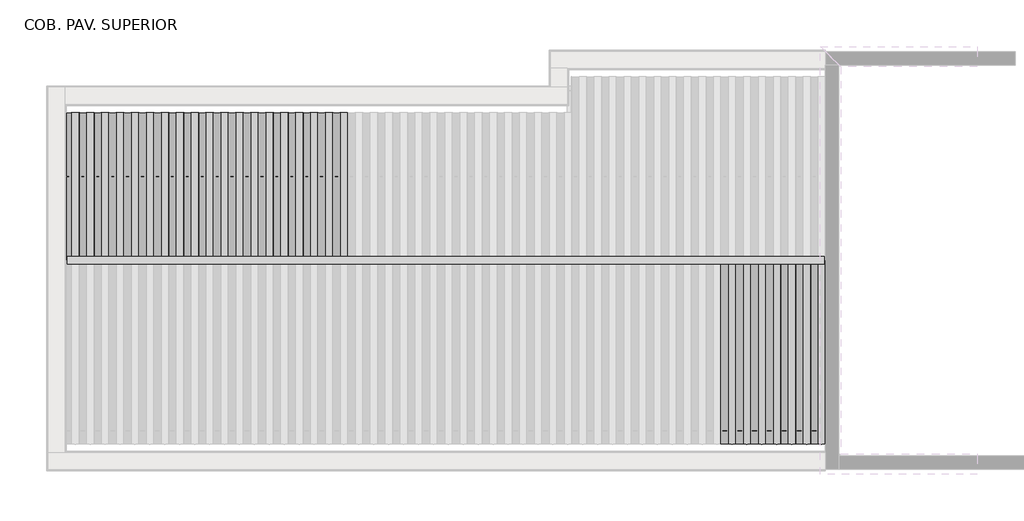
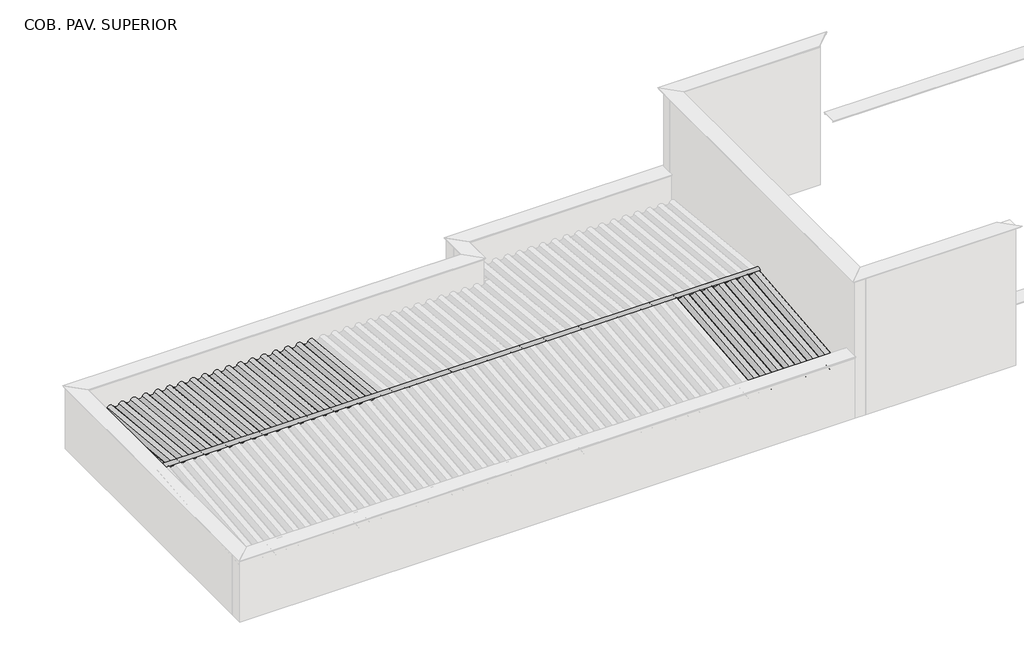
# One storey, part 3 of 7: 37 beams, 7 columns.
"""IFC4 building model written with IfcOpenShell, lengths in millimetres."""

import ifcopenshell
import ifcopenshell.guid

model = None  # the IFC model being written
_history = None  # IfcOwnerHistory: only IFC2X3 demands one
_inside = {}  # id of a spatial element -> (the spatial element, [elements in it])
_under = {}  # id of a project, library or spatial element -> (it, [spatial elements below it])
_declared = {}  # id of a project -> (the project, [libraries it declares])
_typed = {}  # id of a type object -> (the type object, [elements of that type])
_made_of = {}  # id of a material, layer set ... -> (it, [elements and type objects made of it])


def new_model(schema):
    """Start an empty IFC model of exactly this schema.

    Asked for "IFC4X3", IfcOpenShell would pick the latest addendum, in which some entities
    have other attributes; the version numbers below select the first issue.
    IFC2X3 requires an IfcOwnerHistory on every rooted entity: one is made here for all.
    """
    global model, _history
    if schema == "IFC4X3":
        model = ifcopenshell.file(schema_version=(4, 3, 0, 0))
    else:
        model = ifcopenshell.file(schema=schema)
    _inside.clear()
    _under.clear()
    _declared.clear()
    _typed.clear()
    _made_of.clear()
    _history = None
    if model.schema == "IFC2X3":
        org = make("IfcOrganization", Name="unknown")
        user = make(
            "IfcPersonAndOrganization",
            ThePerson=make("IfcPerson", FamilyName="unknown"),
            TheOrganization=org,
        )
        app = make(
            "IfcApplication",
            ApplicationDeveloper=org,
            Version="unknown",
            ApplicationFullName="unknown",
            ApplicationIdentifier="unknown",
        )
        _history = make(
            "IfcOwnerHistory",
            OwningUser=user,
            OwningApplication=app,
            ChangeAction="ADDED",
            CreationDate=0,
        )
    return model


def make(cls, **values):
    """One entity of the class cls with the attributes given. An attribute that is None is left unset."""
    return model.create_entity(
        cls, **{name: value for name, value in values.items() if value is not None}
    )


def rooted(cls, **values):
    """An entity with a GlobalId (a new one), such as an element, a storey or a relation."""
    return make(cls, GlobalId=ifcopenshell.guid.new(), OwnerHistory=_history, **values)


def si_unit(unit_type, name, prefix=None):
    """IfcSIUnit, for example si_unit("LENGTHUNIT", "METRE", prefix="MILLI")."""
    return make("IfcSIUnit", UnitType=unit_type, Prefix=prefix, Name=name)


def assignment(units):
    """IfcUnitAssignment: the units of a project."""
    return None if units is None else make("IfcUnitAssignment", Units=units)


def point(xyz):
    """IfcCartesianPoint."""
    return None if xyz is None else make("IfcCartesianPoint", Coordinates=xyz)


def direction(xyz):
    """IfcDirection."""
    return None if xyz is None else make("IfcDirection", DirectionRatios=xyz)


def frame(location, z_axis=None, x_axis=None):
    """IfcAxis2Placement3D, a coordinate frame: its origin and axes. An axis left out is left unset."""
    return make(
        "IfcAxis2Placement3D",
        Location=point(location),
        Axis=direction(z_axis),
        RefDirection=direction(x_axis),
    )


def frame_2d(location, x_axis=None):
    """IfcAxis2Placement2D, a coordinate frame in the plane: its origin and x axis."""
    return make(
        "IfcAxis2Placement2D", Location=point(location), RefDirection=direction(x_axis)
    )


def origin():
    """The frame at (0, 0, 0) with its axes left unset."""
    return frame((0.0, 0.0, 0.0))


def place(relative_to, where):
    """IfcLocalPlacement: puts the frame where relative to a parent placement (None: the world)."""
    return make(
        "IfcLocalPlacement", PlacementRelTo=relative_to, RelativePlacement=where
    )


def context(
    kind, dimensions, precision=None, world=None, true_north=None, identifier=None
):
    """IfcGeometricRepresentationContext, for example the 3D "Model" context."""
    return make(
        "IfcGeometricRepresentationContext",
        ContextIdentifier=identifier,
        ContextType=kind,
        CoordinateSpaceDimension=dimensions,
        Precision=precision,
        WorldCoordinateSystem=world,
        TrueNorth=true_north,
    )


def project(units=None, contexts=None):
    """IfcProject with its units and contexts."""
    return rooted(
        "IfcProject",
        Name="project",
        RepresentationContexts=contexts,
        UnitsInContext=assignment(units),
    )


def spatial(cls, under=None, at=None, **own):
    """A site, building, storey or space (cls), placed at a placement, below another one or the project."""
    s = rooted(cls, ObjectPlacement=at, **own)
    if under is not None:
        _under.setdefault(under.id(), (under, []))[1].append(s)
    return s


def polyline(points):
    """IfcPolyline through the points."""
    return make("IfcPolyline", Points=[point(p) for p in points])


def circle_curve(where, radius):
    """IfcCircle in the frame where."""
    return make("IfcCircle", Position=where, Radius=radius)


def trimmed(basis, trim1, trim2, sense, master):
    """IfcTrimmedCurve: the piece of a basis curve between two trims."""
    return make(
        "IfcTrimmedCurve",
        BasisCurve=basis,
        Trim1=trim1,
        Trim2=trim2,
        SenseAgreement=sense,
        MasterRepresentation=master,
    )


def segment(curve, same_sense, transition):
    """IfcCompositeCurveSegment."""
    return make(
        "IfcCompositeCurveSegment",
        Transition=transition,
        SameSense=same_sense,
        ParentCurve=curve,
    )


def composite_curve(segments, self_intersect=None):
    """IfcCompositeCurve: segments joined end to end."""
    return make("IfcCompositeCurve", Segments=segments, SelfIntersect=self_intersect)


def outline(outer, holes=None, kind="AREA"):
    """IfcArbitraryClosedProfileDef: a profile drawn as a closed curve; with holes, ...WithVoids."""
    if holes is None:
        return make("IfcArbitraryClosedProfileDef", ProfileType=kind, OuterCurve=outer)
    return make(
        "IfcArbitraryProfileDefWithVoids",
        ProfileType=kind,
        OuterCurve=outer,
        InnerCurves=holes,
    )


def extrude(swept, where, along, depth):
    """IfcExtrudedAreaSolid: the profile swept, set in the frame where, extruded along a direction by depth."""
    return make(
        "IfcExtrudedAreaSolid",
        SweptArea=swept,
        Position=where,
        ExtrudedDirection=direction(along),
        Depth=depth,
    )


def shape(context_of_items, identifier, shape_type, items):
    """IfcShapeRepresentation: the items that make up one representation, for example the "Body"."""
    return make(
        "IfcShapeRepresentation",
        ContextOfItems=context_of_items,
        RepresentationIdentifier=identifier,
        RepresentationType=shape_type,
        Items=items,
    )


def source(mapping_origin, context_of_items, identifier, shape_type, items):
    """IfcRepresentationMap: a shape defined once, which mapped items show again and again."""
    return make(
        "IfcRepresentationMap",
        MappingOrigin=mapping_origin,
        MappedRepresentation=shape(context_of_items, identifier, shape_type, items),
    )


def transform(
    local_origin,
    x_axis=None,
    y_axis=None,
    z_axis=None,
    scale=None,
    scale2=None,
    scale3=None,
    uniform=True,
):
    """IfcCartesianTransformationOperator3D, or its non-uniform kind. x_axis, y_axis, z_axis: its Axis1, 2, 3."""
    if uniform:
        return make(
            "IfcCartesianTransformationOperator3D",
            Axis1=direction(x_axis),
            Axis2=direction(y_axis),
            LocalOrigin=point(local_origin),
            Scale=scale,
            Axis3=direction(z_axis),
        )
    return make(
        "IfcCartesianTransformationOperator3DnonUniform",
        Axis1=direction(x_axis),
        Axis2=direction(y_axis),
        LocalOrigin=point(local_origin),
        Scale=scale,
        Axis3=direction(z_axis),
        Scale2=scale2,
        Scale3=scale3,
    )


def mapped(mapping_source, mapping_target):
    """IfcMappedItem: shows the shape of a source again, moved by a transform."""
    return make(
        "IfcMappedItem", MappingSource=mapping_source, MappingTarget=mapping_target
    )


def made_of(thing, what):
    """Note that an element or type object is made of a material, layer set ...; save() writes the relation."""
    if what is not None:
        _made_of.setdefault(what.id(), (what, []))[1].append(thing)
    return thing


def element(
    cls,
    number,
    at=None,
    inside=None,
    cuts=None,
    type_object=None,
    material=None,
    context=None,
    identifier="Body",
    shape_type=None,
    held_by="IfcProductDefinitionShape",
    body=None,
    shapes=None,
    **own,
):
    """One element of the class cls, such as IfcWall. Its Tag is "e" and its number.

    at: its placement. inside: the storey or other place that contains it. cuts: it is an
    opening in that element (IfcRelVoidsElement). A single representation is given by context,
    identifier, shape_type and body (its items); several are given by shapes. held_by: the class
    of the entity that holds the representations. save() writes the other relations.
    """
    e = rooted(cls, Tag="e%d" % number, ObjectPlacement=at, **own)
    if body is not None:
        shapes = [shape(context, identifier, shape_type, body)]
    if shapes is not None:
        e.Representation = make(held_by, Representations=shapes)
    if inside is not None:
        _inside.setdefault(inside.id(), (inside, []))[1].append(e)
    if cuts is not None:
        rooted(
            "IfcRelVoidsElement", RelatingBuildingElement=cuts, RelatedOpeningElement=e
        )
    if type_object is not None:
        _typed.setdefault(type_object.id(), (type_object, []))[1].append(e)
    return made_of(e, material)


def aggregate(whole, parts):
    """IfcRelAggregates: a whole, such as a stair, and the parts it consists of."""
    return rooted("IfcRelAggregates", RelatingObject=whole, RelatedObjects=parts)


def save(model, path):
    """Write the relations noted so far, then the file.

    IfcRelAggregates (storeys below a building ...), IfcRelContainedInSpatialStructure (elements
    in a storey), IfcRelDefinesByType, IfcRelAssociatesMaterial and IfcRelDeclares: one each for
    every whole, place, type object, material and project.
    """
    for whole, parts in _under.values():
        aggregate(whole, parts)
    for where, things in _inside.values():
        rooted(
            "IfcRelContainedInSpatialStructure",
            RelatedElements=things,
            RelatingStructure=where,
        )
    for kind, things in _typed.values():
        rooted("IfcRelDefinesByType", RelatedObjects=things, RelatingType=kind)
    for what, things in _made_of.values():
        rooted("IfcRelAssociatesMaterial", RelatedObjects=things, RelatingMaterial=what)
    for by, libraries in _declared.values():
        rooted("IfcRelDeclares", RelatingContext=by, RelatedDefinitions=libraries)
    model.write(path)


def cumeeira_telha_ondulada_fibrocimento_4a9e66c1(model_context):
    return source(origin(), model_context, "Body", "SweptSolid", [
        extrude(outline(composite_curve([segment(polyline([(58.3970135, 42.4437972), (53.9055884, 40.2467307)]), True, "CONTINUOUS"), segment(trimmed(circle_curve(frame_2d((-1.6029865, 13.0936483)), 61.7939461), [point((53.9055884, 40.2467307))], [point((-57.1115615, 40.2467307))], True, "CARTESIAN"), True, "CONTINUOUS"), segment(polyline([(-57.1115615, 40.2467307), (-61.6029865, 42.4437972)]), True, "CONTINUOUS"), segment(trimmed(circle_curve(frame_2d((-1.6029865, 13.0936483)), 66.7939461), [point((-61.6029865, 42.4437972))], [point((58.3970135, 42.4437972))], False, "CARTESIAN"), True, "CONTINUOUS")], self_intersect=False)), frame((-6200.0, 0.0, 0.0), z_axis=(1.0, 0.0, 0.0), x_axis=(0.0, 1.0, 0.0)), (0.0, 0.0, 1.0), 12400.0),
    ])


def viga_cumeeira_6x16cm_b61bb166(model_context):
    return source(origin(), model_context, "Body", "SweptSolid", [
        extrude(outline(polyline([(6210.0, 30.0), (6210.0, -30.0), (-6210.0, -30.0), (-6210.0, 30.0), (6210.0, 30.0)])), frame((0.0, 0.0, -80.0), z_axis=(0.0, 0.0, 1.0), x_axis=(1.0, 0.0, 0.0)), (0.0, 0.0, 1.0), 160.0),
    ])


def column_d505325c(model_context):
    return source(origin(), model_context, "Body", "SweptSolid", [
        extrude(outline(polyline([(30.0, 80.0), (30.0, -80.0), (-30.0, -80.0), (-30.0, 80.0), (30.0, 80.0)])), frame((0.0, 0.0, 6710.0), z_axis=(0.0, 0.0, 1.0), x_axis=(1.0, 0.0, 0.0)), (0.0, 0.0, 1.0), 750.0),
    ])


def column_df674f92(model_context):
    return source(origin(), model_context, "Body", "SweptSolid", [
        extrude(outline(polyline([(30.0, 80.0), (30.0, -80.0), (-30.0, -80.0), (-30.0, 80.0), (30.0, 80.0)])), frame((0.0, 0.0, 6710.0), z_axis=(0.0, 0.0, 1.0), x_axis=(1.0, 0.0, 0.0)), (0.0, 0.0, 1.0), 575.0),
    ])


def column_4db371bd(model_context):
    return source(origin(), model_context, "Body", "SweptSolid", [
        extrude(outline(polyline([(30.0, 80.0), (30.0, -80.0), (-30.0, -80.0), (-30.0, 80.0), (30.0, 80.0)])), frame((0.0, 0.0, 6710.0), z_axis=(0.0, 0.0, 1.0), x_axis=(1.0, 0.0, 0.0)), (0.0, 0.0, 1.0), 660.0),
    ])


model = new_model("IFC4")

# Units and contexts
model_context = context("Model", 3, world=origin())
ifc_project = project(units=[si_unit("LENGTHUNIT", "METRE", prefix="MILLI")], contexts=[model_context])

# Site, building, storey
site = spatial("IfcSite", under=ifc_project)
building = spatial("IfcBuilding", under=site)
storey = spatial("IfcBuildingStorey", under=building, Name="COB. PAV. SUPERIOR", Elevation=6650.0)

# Beams
placement = place(None, origin())
element("IfcBeam", 1, ObjectType="Madeira de lei : Berço 6x12cm", at=placement, inside=storey, context=model_context, shape_type="SweptSolid", body=[
    extrude(outline(polyline([(-10679.281307, -7711.5607799), (-10679.281307, -7831.5607799), (-12679.281307, -7831.5607799), (-12679.281307, -7711.5607799), (-10679.281307, -7711.5607799)])), frame((0.0, 0.0, 6650.0), z_axis=(0.0, 0.0, 1.0), x_axis=(1.0, 0.0, 0.0)), (0.0, 0.0, 1.0), 60.0),
])
element("IfcBeam", 2, ObjectType="Madeira de lei : Berço 6x12cm", at=placement, inside=storey, context=model_context, shape_type="SweptSolid", body=[
    extrude(outline(polyline([(-8679.281307, -7711.5607799), (-8679.281307, -7831.5607799), (-10679.281307, -7831.5607799), (-10679.281307, -7711.5607799), (-8679.281307, -7711.5607799)])), frame((0.0, 0.0, 6650.0), z_axis=(0.0, 0.0, 1.0), x_axis=(1.0, 0.0, 0.0)), (0.0, 0.0, 1.0), 60.0),
])
element("IfcBeam", 3, ObjectType="Madeira de lei : Berço 6x12cm", at=placement, inside=storey, context=model_context, shape_type="SweptSolid", body=[
    extrude(outline(polyline([(-6679.281307, -7711.5607799), (-6679.281307, -7831.5607799), (-8679.281307, -7831.5607799), (-8679.281307, -7711.5607799), (-6679.281307, -7711.5607799)])), frame((0.0, 0.0, 6650.0), z_axis=(0.0, 0.0, 1.0), x_axis=(1.0, 0.0, 0.0)), (0.0, 0.0, 1.0), 60.0),
])
element("IfcBeam", 4, ObjectType="Madeira de lei : Berço 6x12cm", at=placement, inside=storey, context=model_context, shape_type="SweptSolid", body=[
    extrude(outline(polyline([(-10679.281307, -6319.8711004), (-10679.281307, -6439.8711004), (-12679.281307, -6439.8711004), (-12679.281307, -6319.8711004), (-10679.281307, -6319.8711004)])), frame((0.0, 0.0, 6650.0), z_axis=(0.0, 0.0, 1.0), x_axis=(1.0, 0.0, 0.0)), (0.0, 0.0, 1.0), 60.0),
])
element("IfcBeam", 5, ObjectType="Madeira de lei : Berço 6x12cm", at=placement, inside=storey, context=model_context, shape_type="SweptSolid", body=[
    extrude(outline(polyline([(-10679.281307, -5488.3211004), (-10679.281307, -5608.3211004), (-12679.281307, -5608.3211004), (-12679.281307, -5488.3211004), (-10679.281307, -5488.3211004)])), frame((0.0, 0.0, 6650.0), z_axis=(0.0, 0.0, 1.0), x_axis=(1.0, 0.0, 0.0)), (0.0, 0.0, 1.0), 60.0),
])
element("IfcBeam", 6, ObjectType="Madeira de lei : Berço 6x12cm", at=placement, inside=storey, context=model_context, shape_type="SweptSolid", body=[
    extrude(outline(polyline([(-8779.281307, -5488.3211004), (-8779.281307, -5608.3211004), (-10679.281307, -5608.3211004), (-10679.281307, -5488.3211004), (-8779.281307, -5488.3211004)])), frame((0.0, 0.0, 6650.0), z_axis=(0.0, 0.0, 1.0), x_axis=(1.0, 0.0, 0.0)), (0.0, 0.0, 1.0), 60.0),
])
element("IfcBeam", 7, ObjectType="Madeira de lei : Berço 6x12cm", at=placement, inside=storey, context=model_context, shape_type="SweptSolid", body=[
    extrude(outline(polyline([(-8779.281307, -6319.8711004), (-8779.281307, -6439.8711004), (-10679.281307, -6439.8711004), (-10679.281307, -6319.8711004), (-8779.281307, -6319.8711004)])), frame((0.0, 0.0, 6650.0), z_axis=(0.0, 0.0, 1.0), x_axis=(1.0, 0.0, 0.0)), (0.0, 0.0, 1.0), 60.0),
])
element("IfcBeam", 8, ObjectType="Madeira de lei : Berço 6x12cm", at=placement, inside=storey, context=model_context, shape_type="SweptSolid", body=[
    extrude(outline(polyline([(-679.281307, -9101.268869), (-679.281307, -9221.268869), (-2679.281307, -9221.268869), (-2679.281307, -9101.268869), (-679.281307, -9101.268869)])), frame((0.0, 0.0, 6650.0), z_axis=(0.0, 0.0, 1.0), x_axis=(1.0, 0.0, 0.0)), (0.0, 0.0, 1.0), 60.0),
])
element("IfcBeam", 9, ObjectType="Madeira de lei : Berço 6x12cm", at=placement, inside=storey, context=model_context, shape_type="SweptSolid", body=[
    extrude(outline(polyline([(-259.281307, -9101.268869), (-259.281307, -9221.268869), (-679.281307, -9221.268869), (-679.281307, -9101.268869), (-259.281307, -9101.268869)])), frame((0.0, 0.0, 6650.0), z_axis=(0.0, 0.0, 1.0), x_axis=(1.0, 0.0, 0.0)), (0.0, 0.0, 1.0), 60.0),
])
cumeeira_telha_ondulada_fibrocimento_shape = cumeeira_telha_ondulada_fibrocimento_4a9e66c1(model_context)
element("IfcBeam", 10, ObjectType="Cumeeira Telha Ondulada : Fibrocimento", at=placement, inside=storey, context=model_context, shape_type="MappedRepresentation", body=[
    mapped(cumeeira_telha_ondulada_fibrocimento_shape, transform((-6459.6793166, -7771.5607799, 7660.6251229), x_axis=(-1.0, 0.0, 0.0), y_axis=(0.0, -1.0, 0.0), z_axis=(0.0, 0.0, 1.0))),
])
element("IfcBeam", 11, ObjectType="Telha Ondulada : Fibrocimento", at=placement, inside=storey, context=model_context, shape_type="SweptSolid", body=[
    extrude(outline(composite_curve([segment(trimmed(circle_curve(frame_2d((0.0, 66.7939461)), 66.7939461), [point((29.3501489, 6.7939461))], [point((29.3501489, 126.7939461))], True, "CARTESIAN"), True, "CONTINUOUS"), segment(polyline([(29.3501489, 126.7939461), (31.5472154, 131.2853711)]), True, "CONTINUOUS"), segment(trimmed(circle_curve(frame_2d((0.0, 66.7939461)), 71.7939461), [point((31.5472154, 131.2853711))], [point((31.5472154, 2.3025211))], False, "CARTESIAN"), True, "CONTINUOUS"), segment(trimmed(circle_curve(frame_2d((58.7002978, -53.2060539)), 61.7939461), [point((31.5472154, 2.3025211))], [point((31.5472154, -108.7146289))], True, "CARTESIAN"), True, "CONTINUOUS"), segment(polyline([(31.5472154, -108.7146289), (29.3501489, -113.2060539)]), True, "CONTINUOUS"), segment(trimmed(circle_curve(frame_2d((58.7002978, -53.2060539)), 66.7939461), [point((29.3501489, -113.2060539))], [point((29.3501489, 6.7939461))], False, "CARTESIAN"), True, "CONTINUOUS")], self_intersect=False)), frame((-1827.3843743, -10781.9594023, 7394.5315886), z_axis=(0.0, 0.9950371902099894, 0.09950371902099743), x_axis=(0.0, 0.09950371902099743, -0.9950371902099894)), (0.0, 0.0, 1.0), 3017.2295147),
])
element("IfcBeam", 12, ObjectType="Telha Ondulada : Fibrocimento", at=placement, inside=storey, context=model_context, shape_type="SweptSolid", body=[
    extrude(outline(composite_curve([segment(trimmed(circle_curve(frame_2d((0.0, 66.7939461)), 66.7939461), [point((29.3501489, 6.7939461))], [point((29.3501489, 126.7939461))], True, "CARTESIAN"), True, "CONTINUOUS"), segment(polyline([(29.3501489, 126.7939461), (31.5472154, 131.2853711)]), True, "CONTINUOUS"), segment(trimmed(circle_curve(frame_2d((0.0, 66.7939461)), 71.7939461), [point((31.5472154, 131.2853711))], [point((31.5472154, 2.3025211))], False, "CARTESIAN"), True, "CONTINUOUS"), segment(trimmed(circle_curve(frame_2d((58.7002978, -53.2060539)), 61.7939461), [point((31.5472154, 2.3025211))], [point((31.5472154, -108.7146289))], True, "CARTESIAN"), True, "CONTINUOUS"), segment(polyline([(31.5472154, -108.7146289), (29.3501489, -113.2060539)]), True, "CONTINUOUS"), segment(trimmed(circle_curve(frame_2d((58.7002978, -53.2060539)), 66.7939461), [point((29.3501489, -113.2060539))], [point((29.3501489, 6.7939461))], False, "CARTESIAN"), True, "CONTINUOUS")], self_intersect=False)), frame((-1582.8843743, -10781.9594023, 7394.5315886), z_axis=(0.0, 0.9950371902099894, 0.0995037190209974), x_axis=(0.0, 0.0995037190209974, -0.9950371902099894)), (0.0, 0.0, 1.0), 3017.2295147),
])
element("IfcBeam", 13, ObjectType="Telha Ondulada : Fibrocimento", at=placement, inside=storey, context=model_context, shape_type="SweptSolid", body=[
    extrude(outline(composite_curve([segment(trimmed(circle_curve(frame_2d((0.0, 66.7939461)), 66.7939461), [point((29.3501489, 6.7939461))], [point((29.3501489, 126.7939461))], True, "CARTESIAN"), True, "CONTINUOUS"), segment(polyline([(29.3501489, 126.7939461), (31.5472154, 131.2853711)]), True, "CONTINUOUS"), segment(trimmed(circle_curve(frame_2d((0.0, 66.7939461)), 71.7939461), [point((31.5472154, 131.2853711))], [point((31.5472154, 2.3025211))], False, "CARTESIAN"), True, "CONTINUOUS"), segment(trimmed(circle_curve(frame_2d((58.7002978, -53.2060539)), 61.7939461), [point((31.5472154, 2.3025211))], [point((31.5472154, -108.7146289))], True, "CARTESIAN"), True, "CONTINUOUS"), segment(polyline([(31.5472154, -108.7146289), (29.3501489, -113.2060539)]), True, "CONTINUOUS"), segment(trimmed(circle_curve(frame_2d((58.7002978, -53.2060539)), 66.7939461), [point((29.3501489, -113.2060539))], [point((29.3501489, 6.7939461))], False, "CARTESIAN"), True, "CONTINUOUS")], self_intersect=False)), frame((-1338.3843743, -10781.9594023, 7394.5315886), z_axis=(0.0, 0.9950371902099894, 0.09950371902099736), x_axis=(0.0, 0.09950371902099736, -0.9950371902099894)), (0.0, 0.0, 1.0), 3017.2295147),
])
element("IfcBeam", 14, ObjectType="Telha Ondulada : Fibrocimento", at=placement, inside=storey, context=model_context, shape_type="SweptSolid", body=[
    extrude(outline(composite_curve([segment(trimmed(circle_curve(frame_2d((0.0, 66.7939461)), 66.7939461), [point((29.3501489, 6.7939461))], [point((29.3501489, 126.7939461))], True, "CARTESIAN"), True, "CONTINUOUS"), segment(polyline([(29.3501489, 126.7939461), (31.5472154, 131.2853711)]), True, "CONTINUOUS"), segment(trimmed(circle_curve(frame_2d((0.0, 66.7939461)), 71.7939461), [point((31.5472154, 131.2853711))], [point((31.5472154, 2.3025211))], False, "CARTESIAN"), True, "CONTINUOUS"), segment(trimmed(circle_curve(frame_2d((58.7002978, -53.2060539)), 61.7939461), [point((31.5472154, 2.3025211))], [point((31.5472154, -108.7146289))], True, "CARTESIAN"), True, "CONTINUOUS"), segment(polyline([(31.5472154, -108.7146289), (29.3501489, -113.2060539)]), True, "CONTINUOUS"), segment(trimmed(circle_curve(frame_2d((58.7002978, -53.2060539)), 66.7939461), [point((29.3501489, -113.2060539))], [point((29.3501489, 6.7939461))], False, "CARTESIAN"), True, "CONTINUOUS")], self_intersect=False)), frame((-1093.8843743, -10781.9594023, 7394.5315886), z_axis=(0.0, 0.9950371902099894, 0.09950371902099743), x_axis=(0.0, 0.09950371902099743, -0.9950371902099894)), (0.0, 0.0, 1.0), 3017.2295147),
])
element("IfcBeam", 15, ObjectType="Telha Ondulada : Fibrocimento", at=placement, inside=storey, context=model_context, shape_type="SweptSolid", body=[
    extrude(outline(composite_curve([segment(trimmed(circle_curve(frame_2d((0.0, 66.7939461)), 66.7939461), [point((29.3501489, 6.7939461))], [point((29.3501489, 126.7939461))], True, "CARTESIAN"), True, "CONTINUOUS"), segment(polyline([(29.3501489, 126.7939461), (31.5472154, 131.2853711)]), True, "CONTINUOUS"), segment(trimmed(circle_curve(frame_2d((0.0, 66.7939461)), 71.7939461), [point((31.5472154, 131.2853711))], [point((31.5472154, 2.3025211))], False, "CARTESIAN"), True, "CONTINUOUS"), segment(trimmed(circle_curve(frame_2d((58.7002978, -53.2060539)), 61.7939461), [point((31.5472154, 2.3025211))], [point((31.5472154, -108.7146289))], True, "CARTESIAN"), True, "CONTINUOUS"), segment(polyline([(31.5472154, -108.7146289), (29.3501489, -113.2060539)]), True, "CONTINUOUS"), segment(trimmed(circle_curve(frame_2d((58.7002978, -53.2060539)), 66.7939461), [point((29.3501489, -113.2060539))], [point((29.3501489, 6.7939461))], False, "CARTESIAN"), True, "CONTINUOUS")], self_intersect=False)), frame((-849.3843743, -10781.9594023, 7394.5315886), z_axis=(0.0, 0.9950371902099894, 0.09950371902099743), x_axis=(0.0, 0.09950371902099743, -0.9950371902099894)), (0.0, 0.0, 1.0), 3017.2295147),
])
element("IfcBeam", 16, ObjectType="Telha Ondulada : Fibrocimento", at=placement, inside=storey, context=model_context, shape_type="SweptSolid", body=[
    extrude(outline(composite_curve([segment(trimmed(circle_curve(frame_2d((0.0, 66.7939461)), 66.7939461), [point((29.3501489, 6.7939461))], [point((29.3501489, 126.7939461))], True, "CARTESIAN"), True, "CONTINUOUS"), segment(polyline([(29.3501489, 126.7939461), (31.5472154, 131.2853711)]), True, "CONTINUOUS"), segment(trimmed(circle_curve(frame_2d((0.0, 66.7939461)), 71.7939461), [point((31.5472154, 131.2853711))], [point((31.5472154, 2.3025211))], False, "CARTESIAN"), True, "CONTINUOUS"), segment(trimmed(circle_curve(frame_2d((58.7002978, -53.2060539)), 61.7939461), [point((31.5472154, 2.3025211))], [point((31.5472154, -108.7146289))], True, "CARTESIAN"), True, "CONTINUOUS"), segment(polyline([(31.5472154, -108.7146289), (29.3501489, -113.2060539)]), True, "CONTINUOUS"), segment(trimmed(circle_curve(frame_2d((58.7002978, -53.2060539)), 66.7939461), [point((29.3501489, -113.2060539))], [point((29.3501489, 6.7939461))], False, "CARTESIAN"), True, "CONTINUOUS")], self_intersect=False)), frame((-604.8843743, -10781.9594023, 7394.5315886), z_axis=(0.0, 0.9950371902099894, 0.09950371902099743), x_axis=(0.0, 0.09950371902099743, -0.9950371902099894)), (0.0, 0.0, 1.0), 3017.2295147),
])
element("IfcBeam", 17, ObjectType="Telha Ondulada : Fibrocimento", at=placement, inside=storey, context=model_context, shape_type="SweptSolid", body=[
    extrude(outline(composite_curve([segment(trimmed(circle_curve(frame_2d((0.0, 66.7939461)), 66.7939461), [point((29.3501489, 6.7939461))], [point((29.3501489, 126.7939461))], True, "CARTESIAN"), True, "CONTINUOUS"), segment(polyline([(29.3501489, 126.7939461), (31.5472154, 131.2853711)]), True, "CONTINUOUS"), segment(trimmed(circle_curve(frame_2d((0.0, 66.7939461)), 71.7939461), [point((31.5472154, 131.2853711))], [point((31.5472154, 2.3025211))], False, "CARTESIAN"), True, "CONTINUOUS"), segment(trimmed(circle_curve(frame_2d((58.7002978, -53.2060539)), 61.7939461), [point((31.5472154, 2.3025211))], [point((31.5472154, -108.7146289))], True, "CARTESIAN"), True, "CONTINUOUS"), segment(polyline([(31.5472154, -108.7146289), (29.3501489, -113.2060539)]), True, "CONTINUOUS"), segment(trimmed(circle_curve(frame_2d((58.7002978, -53.2060539)), 66.7939461), [point((29.3501489, -113.2060539))], [point((29.3501489, 6.7939461))], False, "CARTESIAN"), True, "CONTINUOUS")], self_intersect=False)), frame((-360.3843743, -10781.9594023, 7394.5315886), z_axis=(0.0, 0.9950371902099894, 0.09950371902099743), x_axis=(0.0, 0.09950371902099743, -0.9950371902099894)), (0.0, 0.0, 1.0), 3017.2295147),
])
element("IfcBeam", 18, ObjectType="Telha Ondulada : Fibrocimento", at=placement, inside=storey, context=model_context, shape_type="SweptSolid", body=[
    extrude(outline(composite_curve([segment(trimmed(circle_curve(frame_2d((-58.7002978, -53.2060539)), 66.7939461), [point((-29.3501489, 6.7939461))], [point((-29.3501489, -113.2060539))], False, "CARTESIAN"), True, "CONTINUOUS"), segment(polyline([(-29.3501489, -113.2060539), (-31.5472154, -108.7146289)]), True, "CONTINUOUS"), segment(trimmed(circle_curve(frame_2d((-58.7002978, -53.2060539)), 61.7939461), [point((-31.5472154, -108.7146289))], [point((-31.5472154, 2.3025211))], True, "CARTESIAN"), True, "CONTINUOUS"), segment(trimmed(circle_curve(frame_2d((0.0, 66.7939461)), 71.7939461), [point((-31.5472154, 2.3025211))], [point((-31.5472154, 131.2853711))], False, "CARTESIAN"), True, "CONTINUOUS"), segment(polyline([(-31.5472154, 131.2853711), (-29.3501489, 126.7939461)]), True, "CONTINUOUS"), segment(trimmed(circle_curve(frame_2d((0.0, 66.7939461)), 66.7939461), [point((-29.3501489, 126.7939461))], [point((-29.3501489, 6.7939461))], True, "CARTESIAN"), True, "CONTINUOUS")], self_intersect=False)), frame((-12585.3843743, -5348.1805671, 7453.4315886), z_axis=(0.0, -0.9950371902099893, 0.09950371902099772), x_axis=(0.0, 0.09950371902099772, 0.9950371902099893)), (0.0, 0.0, 1.0), 2425.2918406),
])
element("IfcBeam", 19, ObjectType="Telha Ondulada : Fibrocimento", at=placement, inside=storey, context=model_context, shape_type="SweptSolid", body=[
    extrude(outline(composite_curve([segment(trimmed(circle_curve(frame_2d((-58.7002978, -53.2060539)), 66.7939461), [point((-29.3501489, 6.7939461))], [point((-29.3501489, -113.2060539))], False, "CARTESIAN"), True, "CONTINUOUS"), segment(polyline([(-29.3501489, -113.2060539), (-31.5472154, -108.7146289)]), True, "CONTINUOUS"), segment(trimmed(circle_curve(frame_2d((-58.7002978, -53.2060539)), 61.7939461), [point((-31.5472154, -108.7146289))], [point((-31.5472154, 2.3025211))], True, "CARTESIAN"), True, "CONTINUOUS"), segment(trimmed(circle_curve(frame_2d((0.0, 66.7939461)), 71.7939461), [point((-31.5472154, 2.3025211))], [point((-31.5472154, 131.2853711))], False, "CARTESIAN"), True, "CONTINUOUS"), segment(polyline([(-31.5472154, 131.2853711), (-29.3501489, 126.7939461)]), True, "CONTINUOUS"), segment(trimmed(circle_curve(frame_2d((0.0, 66.7939461)), 66.7939461), [point((-29.3501489, 126.7939461))], [point((-29.3501489, 6.7939461))], True, "CARTESIAN"), True, "CONTINUOUS")], self_intersect=False)), frame((-12340.8843743, -5348.1805671, 7453.4315886), z_axis=(0.0, -0.9950371902099893, 0.09950371902099772), x_axis=(0.0, 0.09950371902099772, 0.9950371902099893)), (0.0, 0.0, 1.0), 2425.2918406),
])
element("IfcBeam", 20, ObjectType="Telha Ondulada : Fibrocimento", at=placement, inside=storey, context=model_context, shape_type="SweptSolid", body=[
    extrude(outline(composite_curve([segment(trimmed(circle_curve(frame_2d((-58.7002978, -53.2060539)), 66.7939461), [point((-29.3501489, 6.7939461))], [point((-29.3501489, -113.2060539))], False, "CARTESIAN"), True, "CONTINUOUS"), segment(polyline([(-29.3501489, -113.2060539), (-31.5472154, -108.7146289)]), True, "CONTINUOUS"), segment(trimmed(circle_curve(frame_2d((-58.7002978, -53.2060539)), 61.7939461), [point((-31.5472154, -108.7146289))], [point((-31.5472154, 2.3025211))], True, "CARTESIAN"), True, "CONTINUOUS"), segment(trimmed(circle_curve(frame_2d((0.0, 66.7939461)), 71.7939461), [point((-31.5472154, 2.3025211))], [point((-31.5472154, 131.2853711))], False, "CARTESIAN"), True, "CONTINUOUS"), segment(polyline([(-31.5472154, 131.2853711), (-29.3501489, 126.7939461)]), True, "CONTINUOUS"), segment(trimmed(circle_curve(frame_2d((0.0, 66.7939461)), 66.7939461), [point((-29.3501489, 126.7939461))], [point((-29.3501489, 6.7939461))], True, "CARTESIAN"), True, "CONTINUOUS")], self_intersect=False)), frame((-12096.3843743, -5348.1805671, 7453.4315886), z_axis=(0.0, -0.9950371902099893, 0.09950371902099768), x_axis=(0.0, 0.09950371902099768, 0.9950371902099893)), (0.0, 0.0, 1.0), 2425.2918406),
])
element("IfcBeam", 21, ObjectType="Telha Ondulada : Fibrocimento", at=placement, inside=storey, context=model_context, shape_type="SweptSolid", body=[
    extrude(outline(composite_curve([segment(trimmed(circle_curve(frame_2d((-58.7002978, -53.2060539)), 66.7939461), [point((-29.3501489, 6.7939461))], [point((-29.3501489, -113.2060539))], False, "CARTESIAN"), True, "CONTINUOUS"), segment(polyline([(-29.3501489, -113.2060539), (-31.5472154, -108.7146289)]), True, "CONTINUOUS"), segment(trimmed(circle_curve(frame_2d((-58.7002978, -53.2060539)), 61.7939461), [point((-31.5472154, -108.7146289))], [point((-31.5472154, 2.3025211))], True, "CARTESIAN"), True, "CONTINUOUS"), segment(trimmed(circle_curve(frame_2d((0.0, 66.7939461)), 71.7939461), [point((-31.5472154, 2.3025211))], [point((-31.5472154, 131.2853711))], False, "CARTESIAN"), True, "CONTINUOUS"), segment(polyline([(-31.5472154, 131.2853711), (-29.3501489, 126.7939461)]), True, "CONTINUOUS"), segment(trimmed(circle_curve(frame_2d((0.0, 66.7939461)), 66.7939461), [point((-29.3501489, 126.7939461))], [point((-29.3501489, 6.7939461))], True, "CARTESIAN"), True, "CONTINUOUS")], self_intersect=False)), frame((-11851.8843743, -5348.1805671, 7453.4315886), z_axis=(0.0, -0.9950371902099893, 0.09950371902099772), x_axis=(0.0, 0.09950371902099772, 0.9950371902099893)), (0.0, 0.0, 1.0), 2425.2918406),
])
element("IfcBeam", 22, ObjectType="Telha Ondulada : Fibrocimento", at=placement, inside=storey, context=model_context, shape_type="SweptSolid", body=[
    extrude(outline(composite_curve([segment(trimmed(circle_curve(frame_2d((-58.7002978, -53.2060539)), 66.7939461), [point((-29.3501489, 6.7939461))], [point((-29.3501489, -113.2060539))], False, "CARTESIAN"), True, "CONTINUOUS"), segment(polyline([(-29.3501489, -113.2060539), (-31.5472154, -108.7146289)]), True, "CONTINUOUS"), segment(trimmed(circle_curve(frame_2d((-58.7002978, -53.2060539)), 61.7939461), [point((-31.5472154, -108.7146289))], [point((-31.5472154, 2.3025211))], True, "CARTESIAN"), True, "CONTINUOUS"), segment(trimmed(circle_curve(frame_2d((0.0, 66.7939461)), 71.7939461), [point((-31.5472154, 2.3025211))], [point((-31.5472154, 131.2853711))], False, "CARTESIAN"), True, "CONTINUOUS"), segment(polyline([(-31.5472154, 131.2853711), (-29.3501489, 126.7939461)]), True, "CONTINUOUS"), segment(trimmed(circle_curve(frame_2d((0.0, 66.7939461)), 66.7939461), [point((-29.3501489, 126.7939461))], [point((-29.3501489, 6.7939461))], True, "CARTESIAN"), True, "CONTINUOUS")], self_intersect=False)), frame((-11607.3843743, -5348.1805671, 7453.4315886), z_axis=(0.0, -0.9950371902099893, 0.09950371902099772), x_axis=(0.0, 0.09950371902099772, 0.9950371902099893)), (0.0, 0.0, 1.0), 2425.2918406),
])
element("IfcBeam", 23, ObjectType="Telha Ondulada : Fibrocimento", at=placement, inside=storey, context=model_context, shape_type="SweptSolid", body=[
    extrude(outline(composite_curve([segment(trimmed(circle_curve(frame_2d((-58.7002978, -53.2060539)), 66.7939461), [point((-29.3501489, 6.7939461))], [point((-29.3501489, -113.2060539))], False, "CARTESIAN"), True, "CONTINUOUS"), segment(polyline([(-29.3501489, -113.2060539), (-31.5472154, -108.7146289)]), True, "CONTINUOUS"), segment(trimmed(circle_curve(frame_2d((-58.7002978, -53.2060539)), 61.7939461), [point((-31.5472154, -108.7146289))], [point((-31.5472154, 2.3025211))], True, "CARTESIAN"), True, "CONTINUOUS"), segment(trimmed(circle_curve(frame_2d((0.0, 66.7939461)), 71.7939461), [point((-31.5472154, 2.3025211))], [point((-31.5472154, 131.2853711))], False, "CARTESIAN"), True, "CONTINUOUS"), segment(polyline([(-31.5472154, 131.2853711), (-29.3501489, 126.7939461)]), True, "CONTINUOUS"), segment(trimmed(circle_curve(frame_2d((0.0, 66.7939461)), 66.7939461), [point((-29.3501489, 126.7939461))], [point((-29.3501489, 6.7939461))], True, "CARTESIAN"), True, "CONTINUOUS")], self_intersect=False)), frame((-11362.8843743, -5348.1805671, 7453.4315886), z_axis=(0.0, -0.9950371902099893, 0.09950371902099768), x_axis=(0.0, 0.09950371902099768, 0.9950371902099893)), (0.0, 0.0, 1.0), 2425.2918406),
])
element("IfcBeam", 24, ObjectType="Telha Ondulada : Fibrocimento", at=placement, inside=storey, context=model_context, shape_type="SweptSolid", body=[
    extrude(outline(composite_curve([segment(trimmed(circle_curve(frame_2d((-58.7002978, -53.2060539)), 66.7939461), [point((-29.3501489, 6.7939461))], [point((-29.3501489, -113.2060539))], False, "CARTESIAN"), True, "CONTINUOUS"), segment(polyline([(-29.3501489, -113.2060539), (-31.5472154, -108.7146289)]), True, "CONTINUOUS"), segment(trimmed(circle_curve(frame_2d((-58.7002978, -53.2060539)), 61.7939461), [point((-31.5472154, -108.7146289))], [point((-31.5472154, 2.3025211))], True, "CARTESIAN"), True, "CONTINUOUS"), segment(trimmed(circle_curve(frame_2d((0.0, 66.7939461)), 71.7939461), [point((-31.5472154, 2.3025211))], [point((-31.5472154, 131.2853711))], False, "CARTESIAN"), True, "CONTINUOUS"), segment(polyline([(-31.5472154, 131.2853711), (-29.3501489, 126.7939461)]), True, "CONTINUOUS"), segment(trimmed(circle_curve(frame_2d((0.0, 66.7939461)), 66.7939461), [point((-29.3501489, 126.7939461))], [point((-29.3501489, 6.7939461))], True, "CARTESIAN"), True, "CONTINUOUS")], self_intersect=False)), frame((-11118.3843743, -5348.1805671, 7453.4315886), z_axis=(0.0, -0.9950371902099893, 0.09950371902099776), x_axis=(0.0, 0.09950371902099776, 0.9950371902099893)), (0.0, 0.0, 1.0), 2425.2918406),
])
element("IfcBeam", 25, ObjectType="Telha Ondulada : Fibrocimento", at=placement, inside=storey, context=model_context, shape_type="SweptSolid", body=[
    extrude(outline(composite_curve([segment(trimmed(circle_curve(frame_2d((-58.7002978, -53.2060539)), 66.7939461), [point((-29.3501489, 6.7939461))], [point((-29.3501489, -113.2060539))], False, "CARTESIAN"), True, "CONTINUOUS"), segment(polyline([(-29.3501489, -113.2060539), (-31.5472154, -108.7146289)]), True, "CONTINUOUS"), segment(trimmed(circle_curve(frame_2d((-58.7002978, -53.2060539)), 61.7939461), [point((-31.5472154, -108.7146289))], [point((-31.5472154, 2.3025211))], True, "CARTESIAN"), True, "CONTINUOUS"), segment(trimmed(circle_curve(frame_2d((0.0, 66.7939461)), 71.7939461), [point((-31.5472154, 2.3025211))], [point((-31.5472154, 131.2853711))], False, "CARTESIAN"), True, "CONTINUOUS"), segment(polyline([(-31.5472154, 131.2853711), (-29.3501489, 126.7939461)]), True, "CONTINUOUS"), segment(trimmed(circle_curve(frame_2d((0.0, 66.7939461)), 66.7939461), [point((-29.3501489, 126.7939461))], [point((-29.3501489, 6.7939461))], True, "CARTESIAN"), True, "CONTINUOUS")], self_intersect=False)), frame((-10873.8843743, -5348.1805671, 7453.4315886), z_axis=(0.0, -0.9950371902099893, 0.09950371902099772), x_axis=(0.0, 0.09950371902099772, 0.9950371902099893)), (0.0, 0.0, 1.0), 2425.2918406),
])
element("IfcBeam", 26, ObjectType="Telha Ondulada : Fibrocimento", at=placement, inside=storey, context=model_context, shape_type="SweptSolid", body=[
    extrude(outline(composite_curve([segment(trimmed(circle_curve(frame_2d((-58.7002978, -53.2060539)), 66.7939461), [point((-29.3501489, 6.7939461))], [point((-29.3501489, -113.2060539))], False, "CARTESIAN"), True, "CONTINUOUS"), segment(polyline([(-29.3501489, -113.2060539), (-31.5472154, -108.7146289)]), True, "CONTINUOUS"), segment(trimmed(circle_curve(frame_2d((-58.7002978, -53.2060539)), 61.7939461), [point((-31.5472154, -108.7146289))], [point((-31.5472154, 2.3025211))], True, "CARTESIAN"), True, "CONTINUOUS"), segment(trimmed(circle_curve(frame_2d((0.0, 66.7939461)), 71.7939461), [point((-31.5472154, 2.3025211))], [point((-31.5472154, 131.2853711))], False, "CARTESIAN"), True, "CONTINUOUS"), segment(polyline([(-31.5472154, 131.2853711), (-29.3501489, 126.7939461)]), True, "CONTINUOUS"), segment(trimmed(circle_curve(frame_2d((0.0, 66.7939461)), 66.7939461), [point((-29.3501489, 126.7939461))], [point((-29.3501489, 6.7939461))], True, "CARTESIAN"), True, "CONTINUOUS")], self_intersect=False)), frame((-10629.3843743, -5348.1805671, 7453.4315886), z_axis=(0.0, -0.9950371902099893, 0.09950371902099772), x_axis=(0.0, 0.09950371902099772, 0.9950371902099893)), (0.0, 0.0, 1.0), 2425.2918406),
])
element("IfcBeam", 27, ObjectType="Telha Ondulada : Fibrocimento", at=placement, inside=storey, context=model_context, shape_type="SweptSolid", body=[
    extrude(outline(composite_curve([segment(trimmed(circle_curve(frame_2d((-58.7002978, -53.2060539)), 66.7939461), [point((-29.3501489, 6.7939461))], [point((-29.3501489, -113.2060539))], False, "CARTESIAN"), True, "CONTINUOUS"), segment(polyline([(-29.3501489, -113.2060539), (-31.5472154, -108.7146289)]), True, "CONTINUOUS"), segment(trimmed(circle_curve(frame_2d((-58.7002978, -53.2060539)), 61.7939461), [point((-31.5472154, -108.7146289))], [point((-31.5472154, 2.3025211))], True, "CARTESIAN"), True, "CONTINUOUS"), segment(trimmed(circle_curve(frame_2d((0.0, 66.7939461)), 71.7939461), [point((-31.5472154, 2.3025211))], [point((-31.5472154, 131.2853711))], False, "CARTESIAN"), True, "CONTINUOUS"), segment(polyline([(-31.5472154, 131.2853711), (-29.3501489, 126.7939461)]), True, "CONTINUOUS"), segment(trimmed(circle_curve(frame_2d((0.0, 66.7939461)), 66.7939461), [point((-29.3501489, 126.7939461))], [point((-29.3501489, 6.7939461))], True, "CARTESIAN"), True, "CONTINUOUS")], self_intersect=False)), frame((-10384.8843743, -5348.1805671, 7453.4315886), z_axis=(0.0, -0.9950371902099893, 0.09950371902099772), x_axis=(0.0, 0.09950371902099772, 0.9950371902099893)), (0.0, 0.0, 1.0), 2425.2918406),
])
element("IfcBeam", 28, ObjectType="Telha Ondulada : Fibrocimento", at=placement, inside=storey, context=model_context, shape_type="SweptSolid", body=[
    extrude(outline(composite_curve([segment(trimmed(circle_curve(frame_2d((-58.7002978, -53.2060539)), 66.7939461), [point((-29.3501489, 6.7939461))], [point((-29.3501489, -113.2060539))], False, "CARTESIAN"), True, "CONTINUOUS"), segment(polyline([(-29.3501489, -113.2060539), (-31.5472154, -108.7146289)]), True, "CONTINUOUS"), segment(trimmed(circle_curve(frame_2d((-58.7002978, -53.2060539)), 61.7939461), [point((-31.5472154, -108.7146289))], [point((-31.5472154, 2.3025211))], True, "CARTESIAN"), True, "CONTINUOUS"), segment(trimmed(circle_curve(frame_2d((0.0, 66.7939461)), 71.7939461), [point((-31.5472154, 2.3025211))], [point((-31.5472154, 131.2853711))], False, "CARTESIAN"), True, "CONTINUOUS"), segment(polyline([(-31.5472154, 131.2853711), (-29.3501489, 126.7939461)]), True, "CONTINUOUS"), segment(trimmed(circle_curve(frame_2d((0.0, 66.7939461)), 66.7939461), [point((-29.3501489, 126.7939461))], [point((-29.3501489, 6.7939461))], True, "CARTESIAN"), True, "CONTINUOUS")], self_intersect=False)), frame((-10140.3843743, -5348.1805671, 7453.4315886), z_axis=(0.0, -0.9950371902099893, 0.09950371902099768), x_axis=(0.0, 0.09950371902099768, 0.9950371902099893)), (0.0, 0.0, 1.0), 2425.2918406),
])
element("IfcBeam", 29, ObjectType="Telha Ondulada : Fibrocimento", at=placement, inside=storey, context=model_context, shape_type="SweptSolid", body=[
    extrude(outline(composite_curve([segment(trimmed(circle_curve(frame_2d((-58.7002978, -53.2060539)), 66.7939461), [point((-29.3501489, 6.7939461))], [point((-29.3501489, -113.2060539))], False, "CARTESIAN"), True, "CONTINUOUS"), segment(polyline([(-29.3501489, -113.2060539), (-31.5472154, -108.7146289)]), True, "CONTINUOUS"), segment(trimmed(circle_curve(frame_2d((-58.7002978, -53.2060539)), 61.7939461), [point((-31.5472154, -108.7146289))], [point((-31.5472154, 2.3025211))], True, "CARTESIAN"), True, "CONTINUOUS"), segment(trimmed(circle_curve(frame_2d((0.0, 66.7939461)), 71.7939461), [point((-31.5472154, 2.3025211))], [point((-31.5472154, 131.2853711))], False, "CARTESIAN"), True, "CONTINUOUS"), segment(polyline([(-31.5472154, 131.2853711), (-29.3501489, 126.7939461)]), True, "CONTINUOUS"), segment(trimmed(circle_curve(frame_2d((0.0, 66.7939461)), 66.7939461), [point((-29.3501489, 126.7939461))], [point((-29.3501489, 6.7939461))], True, "CARTESIAN"), True, "CONTINUOUS")], self_intersect=False)), frame((-9895.8843743, -5348.1805671, 7453.4315886), z_axis=(0.0, -0.9950371902099893, 0.09950371902099772), x_axis=(0.0, 0.09950371902099772, 0.9950371902099893)), (0.0, 0.0, 1.0), 2425.2918406),
])
element("IfcBeam", 30, ObjectType="Telha Ondulada : Fibrocimento", at=placement, inside=storey, context=model_context, shape_type="SweptSolid", body=[
    extrude(outline(composite_curve([segment(trimmed(circle_curve(frame_2d((-58.7002978, -53.2060539)), 66.7939461), [point((-29.3501489, 6.7939461))], [point((-29.3501489, -113.2060539))], False, "CARTESIAN"), True, "CONTINUOUS"), segment(polyline([(-29.3501489, -113.2060539), (-31.5472154, -108.7146289)]), True, "CONTINUOUS"), segment(trimmed(circle_curve(frame_2d((-58.7002978, -53.2060539)), 61.7939461), [point((-31.5472154, -108.7146289))], [point((-31.5472154, 2.3025211))], True, "CARTESIAN"), True, "CONTINUOUS"), segment(trimmed(circle_curve(frame_2d((0.0, 66.7939461)), 71.7939461), [point((-31.5472154, 2.3025211))], [point((-31.5472154, 131.2853711))], False, "CARTESIAN"), True, "CONTINUOUS"), segment(polyline([(-31.5472154, 131.2853711), (-29.3501489, 126.7939461)]), True, "CONTINUOUS"), segment(trimmed(circle_curve(frame_2d((0.0, 66.7939461)), 66.7939461), [point((-29.3501489, 126.7939461))], [point((-29.3501489, 6.7939461))], True, "CARTESIAN"), True, "CONTINUOUS")], self_intersect=False)), frame((-9651.3843743, -5348.1805671, 7453.4315886), z_axis=(0.0, -0.9950371902099893, 0.09950371902099772), x_axis=(0.0, 0.09950371902099772, 0.9950371902099893)), (0.0, 0.0, 1.0), 2425.2918406),
])
element("IfcBeam", 31, ObjectType="Telha Ondulada : Fibrocimento", at=placement, inside=storey, context=model_context, shape_type="SweptSolid", body=[
    extrude(outline(composite_curve([segment(trimmed(circle_curve(frame_2d((-58.7002978, -53.2060539)), 66.7939461), [point((-29.3501489, 6.7939461))], [point((-29.3501489, -113.2060539))], False, "CARTESIAN"), True, "CONTINUOUS"), segment(polyline([(-29.3501489, -113.2060539), (-31.5472154, -108.7146289)]), True, "CONTINUOUS"), segment(trimmed(circle_curve(frame_2d((-58.7002978, -53.2060539)), 61.7939461), [point((-31.5472154, -108.7146289))], [point((-31.5472154, 2.3025211))], True, "CARTESIAN"), True, "CONTINUOUS"), segment(trimmed(circle_curve(frame_2d((0.0, 66.7939461)), 71.7939461), [point((-31.5472154, 2.3025211))], [point((-31.5472154, 131.2853711))], False, "CARTESIAN"), True, "CONTINUOUS"), segment(polyline([(-31.5472154, 131.2853711), (-29.3501489, 126.7939461)]), True, "CONTINUOUS"), segment(trimmed(circle_curve(frame_2d((0.0, 66.7939461)), 66.7939461), [point((-29.3501489, 126.7939461))], [point((-29.3501489, 6.7939461))], True, "CARTESIAN"), True, "CONTINUOUS")], self_intersect=False)), frame((-9406.8843743, -5348.1805671, 7453.4315886), z_axis=(0.0, -0.9950371902099893, 0.09950371902099768), x_axis=(0.0, 0.09950371902099768, 0.9950371902099893)), (0.0, 0.0, 1.0), 2425.2918406),
])
element("IfcBeam", 32, ObjectType="Telha Ondulada : Fibrocimento", at=placement, inside=storey, context=model_context, shape_type="SweptSolid", body=[
    extrude(outline(composite_curve([segment(trimmed(circle_curve(frame_2d((-58.7002978, -53.2060539)), 66.7939461), [point((-29.3501489, 6.7939461))], [point((-29.3501489, -113.2060539))], False, "CARTESIAN"), True, "CONTINUOUS"), segment(polyline([(-29.3501489, -113.2060539), (-31.5472154, -108.7146289)]), True, "CONTINUOUS"), segment(trimmed(circle_curve(frame_2d((-58.7002978, -53.2060539)), 61.7939461), [point((-31.5472154, -108.7146289))], [point((-31.5472154, 2.3025211))], True, "CARTESIAN"), True, "CONTINUOUS"), segment(trimmed(circle_curve(frame_2d((0.0, 66.7939461)), 71.7939461), [point((-31.5472154, 2.3025211))], [point((-31.5472154, 131.2853711))], False, "CARTESIAN"), True, "CONTINUOUS"), segment(polyline([(-31.5472154, 131.2853711), (-29.3501489, 126.7939461)]), True, "CONTINUOUS"), segment(trimmed(circle_curve(frame_2d((0.0, 66.7939461)), 66.7939461), [point((-29.3501489, 126.7939461))], [point((-29.3501489, 6.7939461))], True, "CARTESIAN"), True, "CONTINUOUS")], self_intersect=False)), frame((-9162.3843743, -5348.1805671, 7453.4315886), z_axis=(0.0, -0.9950371902099893, 0.09950371902099776), x_axis=(0.0, 0.09950371902099776, 0.9950371902099893)), (0.0, 0.0, 1.0), 2425.2918406),
])
element("IfcBeam", 33, ObjectType="Telha Ondulada : Fibrocimento", at=placement, inside=storey, context=model_context, shape_type="SweptSolid", body=[
    extrude(outline(composite_curve([segment(trimmed(circle_curve(frame_2d((-58.7002978, -53.2060539)), 66.7939461), [point((-29.3501489, 6.7939461))], [point((-29.3501489, -113.2060539))], False, "CARTESIAN"), True, "CONTINUOUS"), segment(polyline([(-29.3501489, -113.2060539), (-31.5472154, -108.7146289)]), True, "CONTINUOUS"), segment(trimmed(circle_curve(frame_2d((-58.7002978, -53.2060539)), 61.7939461), [point((-31.5472154, -108.7146289))], [point((-31.5472154, 2.3025211))], True, "CARTESIAN"), True, "CONTINUOUS"), segment(trimmed(circle_curve(frame_2d((0.0, 66.7939461)), 71.7939461), [point((-31.5472154, 2.3025211))], [point((-31.5472154, 131.2853711))], False, "CARTESIAN"), True, "CONTINUOUS"), segment(polyline([(-31.5472154, 131.2853711), (-29.3501489, 126.7939461)]), True, "CONTINUOUS"), segment(trimmed(circle_curve(frame_2d((0.0, 66.7939461)), 66.7939461), [point((-29.3501489, 126.7939461))], [point((-29.3501489, 6.7939461))], True, "CARTESIAN"), True, "CONTINUOUS")], self_intersect=False)), frame((-8917.8843743, -5348.1805671, 7453.4315886), z_axis=(0.0, -0.9950371902099893, 0.09950371902099772), x_axis=(0.0, 0.09950371902099772, 0.9950371902099893)), (0.0, 0.0, 1.0), 2425.2918406),
])
element("IfcBeam", 34, ObjectType="Telha Ondulada : Fibrocimento", at=placement, inside=storey, context=model_context, shape_type="SweptSolid", body=[
    extrude(outline(composite_curve([segment(trimmed(circle_curve(frame_2d((-58.7002978, -53.2060539)), 66.7939461), [point((-29.3501489, 6.7939461))], [point((-29.3501489, -113.2060539))], False, "CARTESIAN"), True, "CONTINUOUS"), segment(polyline([(-29.3501489, -113.2060539), (-31.5472154, -108.7146289)]), True, "CONTINUOUS"), segment(trimmed(circle_curve(frame_2d((-58.7002978, -53.2060539)), 61.7939461), [point((-31.5472154, -108.7146289))], [point((-31.5472154, 2.3025211))], True, "CARTESIAN"), True, "CONTINUOUS"), segment(trimmed(circle_curve(frame_2d((0.0, 66.7939461)), 71.7939461), [point((-31.5472154, 2.3025211))], [point((-31.5472154, 131.2853711))], False, "CARTESIAN"), True, "CONTINUOUS"), segment(polyline([(-31.5472154, 131.2853711), (-29.3501489, 126.7939461)]), True, "CONTINUOUS"), segment(trimmed(circle_curve(frame_2d((0.0, 66.7939461)), 66.7939461), [point((-29.3501489, 126.7939461))], [point((-29.3501489, 6.7939461))], True, "CARTESIAN"), True, "CONTINUOUS")], self_intersect=False)), frame((-8673.3843743, -5348.1805671, 7453.4315886), z_axis=(0.0, -0.9950371902099893, 0.09950371902099772), x_axis=(0.0, 0.09950371902099772, 0.9950371902099893)), (0.0, 0.0, 1.0), 2425.2918406),
])
element("IfcBeam", 35, ObjectType="Telha Ondulada : Fibrocimento", at=placement, inside=storey, context=model_context, shape_type="SweptSolid", body=[
    extrude(outline(composite_curve([segment(trimmed(circle_curve(frame_2d((-58.7002978, -53.2060539)), 66.7939461), [point((-29.3501489, 6.7939461))], [point((-29.3501489, -113.2060539))], False, "CARTESIAN"), True, "CONTINUOUS"), segment(polyline([(-29.3501489, -113.2060539), (-31.5472154, -108.7146289)]), True, "CONTINUOUS"), segment(trimmed(circle_curve(frame_2d((-58.7002978, -53.2060539)), 61.7939461), [point((-31.5472154, -108.7146289))], [point((-31.5472154, 2.3025211))], True, "CARTESIAN"), True, "CONTINUOUS"), segment(trimmed(circle_curve(frame_2d((0.0, 66.7939461)), 71.7939461), [point((-31.5472154, 2.3025211))], [point((-31.5472154, 131.2853711))], False, "CARTESIAN"), True, "CONTINUOUS"), segment(polyline([(-31.5472154, 131.2853711), (-29.3501489, 126.7939461)]), True, "CONTINUOUS"), segment(trimmed(circle_curve(frame_2d((0.0, 66.7939461)), 66.7939461), [point((-29.3501489, 126.7939461))], [point((-29.3501489, 6.7939461))], True, "CARTESIAN"), True, "CONTINUOUS")], self_intersect=False)), frame((-8428.8843743, -5348.1805671, 7453.4315886), z_axis=(0.0, -0.9950371902099893, 0.09950371902099772), x_axis=(0.0, 0.09950371902099772, 0.9950371902099893)), (0.0, 0.0, 1.0), 2425.2918406),
])
element("IfcBeam", 36, ObjectType="Telha Ondulada : Fibrocimento", at=placement, inside=storey, context=model_context, shape_type="SweptSolid", body=[
    extrude(outline(composite_curve([segment(trimmed(circle_curve(frame_2d((-58.7002978, -53.2060539)), 66.7939461), [point((-29.3501489, 6.7939461))], [point((-29.3501489, -113.2060539))], False, "CARTESIAN"), True, "CONTINUOUS"), segment(polyline([(-29.3501489, -113.2060539), (-31.5472154, -108.7146289)]), True, "CONTINUOUS"), segment(trimmed(circle_curve(frame_2d((-58.7002978, -53.2060539)), 61.7939461), [point((-31.5472154, -108.7146289))], [point((-31.5472154, 2.3025211))], True, "CARTESIAN"), True, "CONTINUOUS"), segment(trimmed(circle_curve(frame_2d((0.0, 66.7939461)), 71.7939461), [point((-31.5472154, 2.3025211))], [point((-31.5472154, 131.2853711))], False, "CARTESIAN"), True, "CONTINUOUS"), segment(polyline([(-31.5472154, 131.2853711), (-29.3501489, 126.7939461)]), True, "CONTINUOUS"), segment(trimmed(circle_curve(frame_2d((0.0, 66.7939461)), 66.7939461), [point((-29.3501489, 126.7939461))], [point((-29.3501489, 6.7939461))], True, "CARTESIAN"), True, "CONTINUOUS")], self_intersect=False)), frame((-8184.3843743, -5348.1805671, 7453.4315886), z_axis=(0.0, -0.9950371902099893, 0.09950371902099768), x_axis=(0.0, 0.09950371902099768, 0.9950371902099893)), (0.0, 0.0, 1.0), 2425.2918406),
])
viga_cumeeira_6x16cm_shape = viga_cumeeira_6x16cm_b61bb166(model_context)
element("IfcBeam", 37, ObjectType="Madeira de lei : Viga Cumeeira 6x16cm", at=placement, inside=storey, context=model_context, shape_type="MappedRepresentation", body=[
    mapped(viga_cumeeira_6x16cm_shape, transform((-6464.281307, -7771.5607799, 7540.0), x_axis=(1.0, 0.0, 0.0), y_axis=(0.0, 1.0, 0.0), z_axis=(0.0, 0.0, 1.0))),
])

# Columns
column_shape = column_d505325c(model_context)
element("IfcColumn", 38, ObjectType="Madeira de lei-Coluna : Pontalete 6X16cm", at=placement, inside=storey, context=model_context, shape_type="MappedRepresentation", body=[
    mapped(column_shape, transform((-9679.281307, -7771.5607799, 0.0), x_axis=(0.0, 1.0, 0.0), y_axis=(-1.0, 0.0, 0.0), z_axis=(0.0, 0.0, 1.0))),
])
element("IfcColumn", 39, ObjectType="Madeira de lei-Coluna : Pontalete 6X16cm", at=placement, inside=storey, context=model_context, shape_type="MappedRepresentation", body=[
    mapped(column_shape, transform((-7679.281307, -7771.5607799, 0.0), x_axis=(0.0, 1.0, 0.0), y_axis=(-1.0, 0.0, 0.0), z_axis=(0.0, 0.0, 1.0))),
])
column_2_shape = column_df674f92(model_context)
element("IfcColumn", 40, ObjectType="Madeira de lei-Coluna : Pontalete 6X16cm", at=placement, inside=storey, context=model_context, shape_type="MappedRepresentation", body=[
    mapped(column_2_shape, transform((-11679.281307, -5548.3211004, 0.0), x_axis=(0.0, 1.0, 0.0), y_axis=(-1.0, 0.0, 0.0), z_axis=(0.0, 0.0, 1.0))),
])
element("IfcColumn", 41, ObjectType="Madeira de lei-Coluna : Pontalete 6X16cm", at=placement, inside=storey, context=model_context, shape_type="MappedRepresentation", body=[
    mapped(column_2_shape, transform((-9679.281307, -5548.3211004, 0.0), x_axis=(0.0, 1.0, 0.0), y_axis=(-1.0, 0.0, 0.0), z_axis=(0.0, 0.0, 1.0))),
])
column_3_shape = column_4db371bd(model_context)
element("IfcColumn", 42, ObjectType="Madeira de lei-Coluna : Pontalete 6X16cm", at=placement, inside=storey, context=model_context, shape_type="MappedRepresentation", body=[
    mapped(column_3_shape, transform((-11679.281307, -6379.8711004, 0.0), x_axis=(0.0, 1.0, 0.0), y_axis=(-1.0, 0.0, 0.0), z_axis=(0.0, 0.0, 1.0))),
])
element("IfcColumn", 43, ObjectType="Madeira de lei-Coluna : Pontalete 6X16cm", at=placement, inside=storey, context=model_context, shape_type="MappedRepresentation", body=[
    mapped(column_3_shape, transform((-9679.281307, -6379.8711004, 0.0), x_axis=(0.0, 1.0, 0.0), y_axis=(-1.0, 0.0, 0.0), z_axis=(0.0, 0.0, 1.0))),
])
element("IfcColumn", 44, ObjectType="Madeira de lei-Coluna : Pontalete 6X16cm", at=placement, inside=storey, context=model_context, shape_type="MappedRepresentation", body=[
    mapped(column_3_shape, transform((-1679.281307, -9161.268869, 0.0), x_axis=(0.0, 1.0, 0.0), y_axis=(-1.0, 0.0, 0.0), z_axis=(0.0, 0.0, 1.0))),
])

save(model, "model.ifc")

# Revit data of these elements
# Type "Madeira de lei : Berço 6x12cm"
#   A = 0.02 m²
#   Length [instance default] = 1.524 m
#   b = 0.06 m
#   d = 0.12 m
#   Structural Material [instance default] = none
#   Assembly Code = ""
# Type "Cumeeira Telha Ondulada : Fibrocimento"
#   Cost = 5
#   Length [instance default] = 1.524 m
#   b = 0.07 m
#   h = 0.16 m
#   Structural Material = .TELHA DE FIBROCIMENTO
#   Assembly Code = ""
# Type "Telha Ondulada : Fibrocimento"
#   Description = "TELHA ONDULADA FIBROCIMENTO"
#   Cost = 5
#   Length [instance default] = 1.524 m
#   b = 0.07 m
#   h = 0.16 m
#   Structural Material = .TELHA DE FIBROCIMENTO
#   Assembly Code = ""
# Type "Madeira de lei : Viga Cumeeira 6x16cm"
#   A = 0.02 m²
#   Length [instance default] = 1.524 m
#   b = 0.06 m
#   d = 0.16 m
#   Structural Material [instance default] = none
#   Assembly Code = ""
# Type "Madeira de lei-Coluna : Pontalete 6X16cm"
#   A = 0.01952 m²
#   b = 0.06 m
#   d = 0.16 m
#   Structural Material [instance default] = none
#   Assembly Code = ""
# Elements 1, 2, 3, 4, 5, 6, 7, 8, 9 (IfcBeam, "Madeira de lei : Berço 6x12cm")
#   Comments = ""
#   Structural Material = .MADEIRAMENTO
#   Phase Created = CC_PE
#   Materials on its faces: ".MADEIRAMENTO"
# Element 10 (IfcBeam, "Cumeeira Telha Ondulada : Fibrocimento")
#   Comments = ""
#   Phase Created = CC_PE
#   Materials on its faces: ".TELHA DE FIBROCIMENTO"
# Elements 11, 12, 13, 14, 15, 16, 17, 18, 19, 20, 21, 22, 23, 24, 25, 26, 27, 28, 29, 30, 31, 32, 33, 34, 35, 36 (IfcBeam, "Telha Ondulada : Fibrocimento")
#   Phase Created = CC_PE
#   Materials on its faces: ".TELHA DE FIBROCIMENTO"
# Element 37 (IfcBeam, "Madeira de lei : Viga Cumeeira 6x16cm")
#   Comments = ""
#   Structural Material = .MADEIRAMENTO
#   Phase Created = CC_PE
#   Materials on its faces: ".MADEIRAMENTO"
# Elements 38, 39, 40, 41, 42, 43, 44 (IfcColumn, "Madeira de lei-Coluna : Pontalete 6X16cm")
#   Comments = ""
#   Structural Material = .MADEIRAMENTO
#   Phase Created = CC_PE
#   Materials on its faces: ".MADEIRAMENTO"
# Materials
#   ".TELHA DE FIBROCIMENTO": class "CC_TELHADO", colour RGB 77 77 76, transparency 0, Description = "TELHA ONDULADA FIBROCIMENTO", Cost = 0
#   ".MADEIRAMENTO": class ".CC_MADEIRAS", colour RGB 212 179 113, transparency 0, Cost = 0
